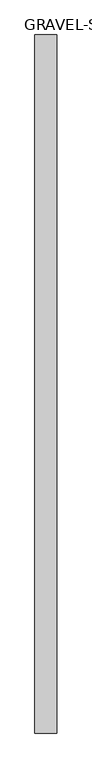
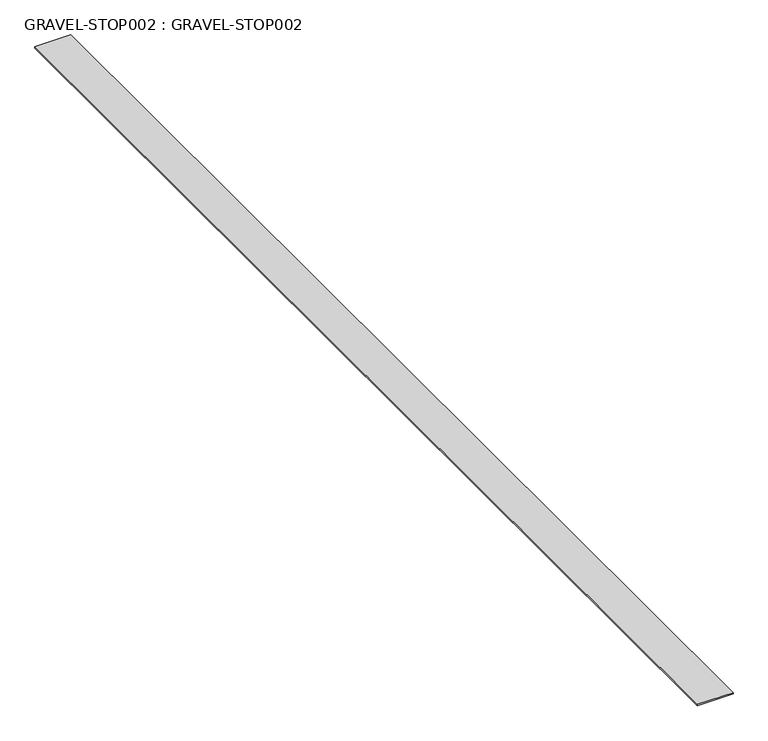
"""IFC4 building model written with IfcOpenShell, lengths in millimetres: proxy geometry, GRAVEL-STOP002 : GRAVEL-STOP002."""

from ifc_helpers import new_model, si_unit, frame, origin, place, context, project, spatial, polyline, outline, extrude, source, transform, mapped, element, save


def gravel_stop002_gravel_stop002_735a63bd(model_context):
    return source(origin(), model_context, "Body", "SweptSolid", [
        extrude(outline(polyline([(-4430.8949897, -1065.5906573), (-4493.2230977, -1065.5906573), (-4493.2230977, 934.6593427), (-4430.8949897, 934.6593427), (-4430.8949897, -1065.5906573)])), frame((0.0, 0.0, 40252.8572765), z_axis=(0.0, 0.0, 1.0), x_axis=(1.0, 0.0, 0.0)), (0.0, 0.0, 1.0), 2.3397091),
    ])


if __name__ == "__main__":
    model = new_model("IFC4")
    model_context = context("Model", 3, world=origin())
    ifc_project = project(units=[si_unit("LENGTHUNIT", "METRE", prefix="MILLI")], contexts=[model_context])
    site = spatial("IfcSite", under=ifc_project)
    building = spatial("IfcBuilding", under=site)
    placement = place(None, origin())
    gravel_stop002_gravel_stop002_shape = gravel_stop002_gravel_stop002_735a63bd(model_context)
    element("IfcBuildingElementProxy", 1, Name="GRAVEL-STOP002 : GRAVEL-STOP002", ObjectType="GRAVEL-STOP002 : GRAVEL-STOP002", at=placement, inside=building, context=model_context, shape_type="MappedRepresentation", body=[
        mapped(gravel_stop002_gravel_stop002_shape, transform((0.0, 0.0, 0.0), x_axis=(1.0, 0.0, 0.0), y_axis=(0.0, 1.0, 0.0), z_axis=(0.0, 0.0, 1.0))),
    ])
    save(model, "model.ifc")

# Revit data of these elements
# Type "GRAVEL-STOP002 : GRAVEL-STOP002"
#   NameOverride = "GRAVEL-STOP002"
# Element 1 (IfcBuildingElementProxy, "GRAVEL-STOP002 : GRAVEL-STOP002")
#   Materials on its faces: "METAL FLASHING"
# Materials
#   "METAL FLASHING": class "Unassigned", colour RGB 128 128 128, transparency 0
